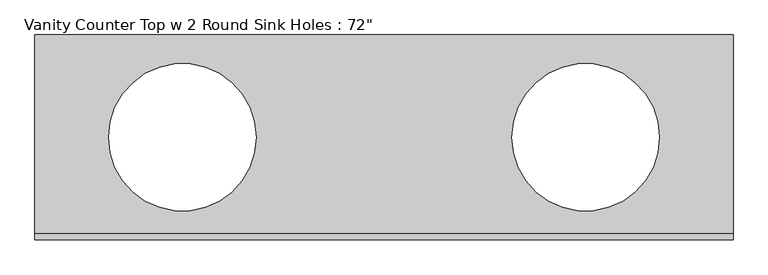
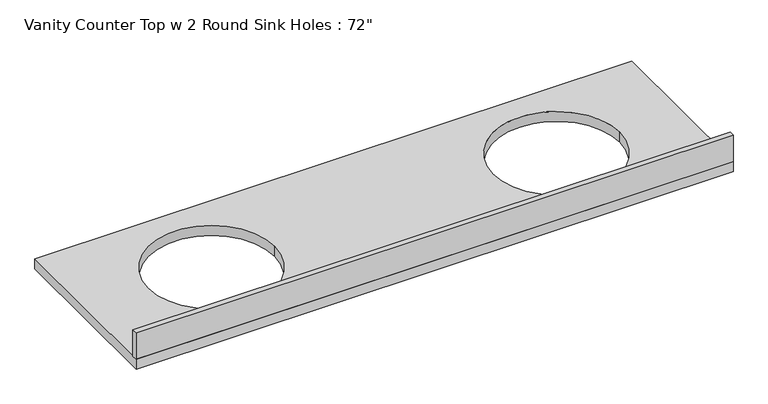
"""IFC4 building model written with IfcOpenShell, lengths in millimetres: furniture geometry."""

from ifc_helpers import new_model, si_unit, point, frame, frame_2d, origin, place, context, project, spatial, polyline, circle_curve, trimmed, segment, composite_curve, outline, extrude, source, transform, mapped, element, save


def furniture_10a5812a(model_context):
    return source(origin(), model_context, "Body", "SweptSolid", [
        extrude(outline(polyline([(-1327.4622951, 0.0), (-1327.4622951, 19.05), (837.8877049, 19.05), (837.8877049, 0.0), (-1327.4622951, 0.0)])), frame((0.0, 0.0, 787.4), z_axis=(0.0, 0.0, 1.0), x_axis=(1.0, 0.0, 0.0)), (0.0, 0.0, 1.0), 101.6),
        extrude(outline(polyline([(837.8877049, 0.0), (-1327.4622951, 0.0), (-1327.4622951, 635.0), (837.8877049, 635.0), (837.8877049, 0.0)]), holes=[composite_curve([segment(trimmed(circle_curve(frame_2d((-870.2622951, 317.5)), 228.6), [point((-1098.8622951, 317.5))], [point((-641.6622951, 317.5))], True, "CARTESIAN"), True, "CONTINUOUS"), segment(trimmed(circle_curve(frame_2d((-870.2622951, 317.5)), 228.6), [point((-641.6622951, 317.5))], [point((-1098.8622951, 317.5))], True, "CARTESIAN"), True, "CONTINUOUS")], self_intersect=False), composite_curve([segment(trimmed(circle_curve(frame_2d((380.6877049, 317.5)), 228.6), [point((152.0877049, 317.5))], [point((609.2877049, 317.5))], True, "CARTESIAN"), True, "CONTINUOUS"), segment(trimmed(circle_curve(frame_2d((380.6877049, 317.5)), 228.6), [point((609.2877049, 317.5))], [point((152.0877049, 317.5))], True, "CARTESIAN"), True, "CONTINUOUS")], self_intersect=False)]), frame((0.0, 0.0, 749.3), z_axis=(0.0, 0.0, 1.0), x_axis=(1.0, 0.0, 0.0)), (0.0, 0.0, 1.0), 38.1),
    ])


if __name__ == "__main__":
    model = new_model("IFC4")
    model_context = context("Model", 3, world=origin())
    ifc_project = project(units=[si_unit("LENGTHUNIT", "METRE", prefix="MILLI")], contexts=[model_context])
    site = spatial("IfcSite", under=ifc_project)
    building = spatial("IfcBuilding", under=site)
    placement = place(None, origin())
    furniture_shape = furniture_10a5812a(model_context)
    element("IfcFurniture", 1, ObjectType="Vanity Counter Top w 2 Round Sink Holes : 72\"", at=placement, inside=building, context=model_context, shape_type="MappedRepresentation", body=[
        mapped(furniture_shape, transform((0.0, 0.0, 0.0), x_axis=(1.0, 0.0, 0.0), y_axis=(0.0, 1.0, 0.0), z_axis=(0.0, 0.0, 1.0))),
    ])
    save(model, "model.ifc")

# Revit data of these elements
# Type "Vanity Counter Top w 2 Round Sink Holes : 72\""
#   Assembly Code = "C1030400"
#   Sink Location Right = 1' - 6"
#   Counter Thickness = 0' - 1 1/2"
#   Depth = 2' - 1"
#   Height = 2' - 7"
#   Length [instance default] = 6' - 0"
#   Sink Location Left [instance default] = 1' - 6"
#   Sink Location To Wall [instance default] = 0' - 4"
#   Sink Opening Width [instance default] = 1' - 5"
#   Counter Top = Counter Top
# Element 1 (IfcFurniture, "Vanity Counter Top w 2 Round Sink Holes : 72\"")
#   Length = 7' - 1 1/4"
#   Materials on its faces: "Counter Top"
# Materials
#   "Counter Top": class "Wood", colour RGB 226 177 128, transparency 0
